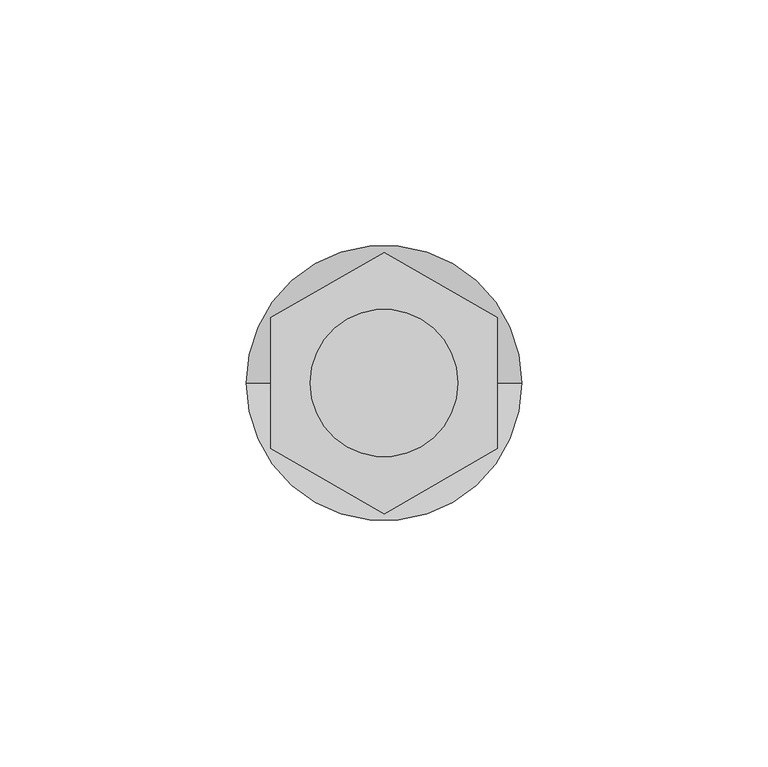
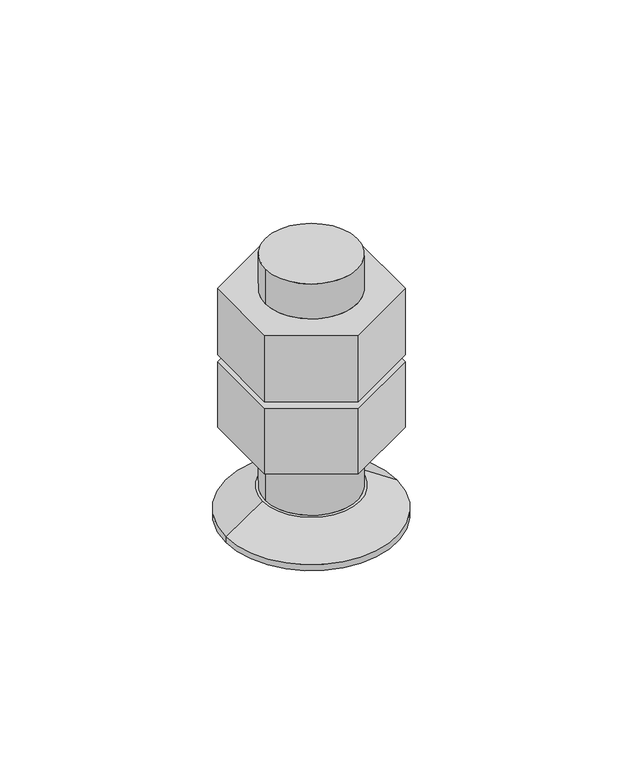
"""IFC4 building model written with IfcOpenShell, lengths in millimetres: fastener geometry, Bolt HPM-L : 30/L_mk."""

from ifc_helpers import new_model, si_unit, frame, origin, origin_with_axes, place, context, project, spatial, polyline, circle_curve, source, transform, mapped, element, save
from ifc_brep_helpers import plane_surface, cylinder_surface, revolved_surface, advanced_brep


def fastener_9f417b6c(model_context):
    return source(origin(), model_context, "Body", "AdvancedBrep", [
        advanced_brep(
        [(-23.0, -13.2790562, 22.7), (0.0, -26.5581124, 22.7), (23.0, -13.2790562, 22.7), (23.0, 13.2790562, 22.7), (0.0, 26.5581124, 22.7), (-23.0, 13.2790562, 22.7), (15.0, 0.0, 22.7), (-15.0, 0.0, 22.7), (-23.0, -13.2790562, 0.0), (-23.0, 13.2790562, 0.0), (0.0, 26.5581124, 0.0), (23.0, 13.2790562, 0.0), (23.0, -13.2790562, 0.0), (0.0, -26.5581124, 0.0), (-15.0, 0.0, 0.0), (15.0, 0.0, 0.0), (-15.0, 0.0, 60.0), (15.0, 0.0, 60.0), (15.0, 0.0, 48.0), (-15.0, 0.0, 48.0), (-15.0, 0.0, 25.0), (15.0, 0.0, 25.0), (15.0, 0.0, -20.0), (-15.0, 0.0, -20.0), (-23.0, -13.2790562, 48.0), (0.0, -26.5581124, 48.0), (23.0, -13.2790562, 48.0), (23.0, 13.2790562, 48.0), (0.0, 26.5581124, 48.0), (-23.0, 13.2790562, 48.0), (-23.0, -13.2790562, 25.0), (-23.0, 13.2790562, 25.0), (0.0, 26.5581124, 25.0), (23.0, 13.2790562, 25.0), (23.0, -13.2790562, 25.0), (0.0, -26.5581124, 25.0), (-28.0, 0.0, -30.0), (-28.0, 0.0, -28.0), (28.0, 0.0, -28.0), (28.0, 0.0, -30.0), (-16.0, 0.0, -20.0), (16.0, 0.0, -20.0)],
        [
            (0, 1),
            (1, 2),
            (2, 3),
            (3, 4),
            (4, 5),
            (5, 0),
            (6, 7, circle_curve(frame((0.0, 0.0, 22.7), z_axis=(0.0, 0.0, -1.0), x_axis=(1.0, 0.0, 0.0)), 15.0)),
            (7, 6, circle_curve(frame((0.0, 0.0, 22.7), z_axis=(0.0, 0.0, -1.0), x_axis=(1.0, 0.0, 0.0)), 15.0)),
            (8, 9),
            (9, 10),
            (10, 11),
            (11, 12),
            (12, 13),
            (13, 8),
            (14, 15, circle_curve(origin_with_axes(), 15.0)),
            (15, 14, circle_curve(origin_with_axes(), 15.0)),
            (5, 9),
            (8, 0),
            (4, 10),
            (3, 11),
            (2, 12),
            (1, 13),
            (16, 17, circle_curve(frame((0.0, 0.0, 60.0), z_axis=(0.0, 0.0, 1.0), x_axis=(1.0, 0.0, 0.0)), 15.0)),
            (17, 16, circle_curve(frame((0.0, 0.0, 60.0), z_axis=(0.0, 0.0, 1.0), x_axis=(1.0, 0.0, 0.0)), 15.0)),
            (17, 18),
            (18, 19, circle_curve(frame((0.0, 0.0, 48.0), z_axis=(0.0, 0.0, 1.0), x_axis=(1.0, 0.0, 0.0)), 15.0)),
            (19, 16),
            (7, 20),
            (20, 21, circle_curve(frame((0.0, 0.0, 25.0), z_axis=(0.0, 0.0, -1.0), x_axis=(1.0, 0.0, 0.0)), 15.0)),
            (21, 6),
            (15, 22),
            (22, 23, circle_curve(frame((0.0, 0.0, -20.0), z_axis=(0.0, 0.0, 1.0), x_axis=(1.0, 0.0, 0.0)), 15.0)),
            (23, 14),
            (19, 18, circle_curve(frame((0.0, 0.0, 48.0), z_axis=(0.0, 0.0, 1.0), x_axis=(1.0, 0.0, 0.0)), 15.0)),
            (21, 20, circle_curve(frame((0.0, 0.0, 25.0), z_axis=(0.0, 0.0, -1.0), x_axis=(1.0, 0.0, 0.0)), 15.0)),
            (23, 22, circle_curve(frame((0.0, 0.0, -20.0), z_axis=(0.0, 0.0, 1.0), x_axis=(1.0, 0.0, 0.0)), 15.0)),
            (24, 25),
            (25, 26),
            (26, 27),
            (27, 28),
            (28, 29),
            (29, 24),
            (30, 31),
            (31, 32),
            (32, 33),
            (33, 34),
            (34, 35),
            (35, 30),
            (29, 31),
            (30, 24),
            (28, 32),
            (27, 33),
            (26, 34),
            (25, 35),
            (36, 37),
            (37, 38, circle_curve(frame((0.0, 0.0, -28.0), z_axis=(0.0, 0.0, -1.0), x_axis=(1.0, 0.0, 0.0)), 28.0)),
            (38, 39),
            (39, 36, circle_curve(frame((0.0, 0.0, -30.0), z_axis=(0.0, 0.0, 1.0), x_axis=(1.0, 0.0, 0.0)), 28.0)),
            (38, 37, circle_curve(frame((0.0, 0.0, -28.0), z_axis=(0.0, 0.0, -1.0), x_axis=(1.0, 0.0, 0.0)), 28.0)),
            (36, 39, circle_curve(frame((0.0, 0.0, -30.0), z_axis=(0.0, 0.0, 1.0), x_axis=(1.0, 0.0, 0.0)), 28.0)),
            (40, 41, circle_curve(frame((0.0, 0.0, -20.0), z_axis=(0.0, 0.0, -1.0), x_axis=(1.0, 0.0, 0.0)), 16.0)),
            (41, 38),
            (37, 40),
            (41, 40, circle_curve(frame((0.0, 0.0, -20.0), z_axis=(0.0, 0.0, -1.0), x_axis=(-1.0, 0.0, 0.0)), 16.0)),
        ],
        [
            plane_surface(frame((-23.0, -13.2790562, 22.7), z_axis=(0.0, 0.0, 1.0), x_axis=(0.0, 1.0, 0.0))),
            plane_surface(frame((-23.0, -13.2790562, 0.0), z_axis=(0.0, 0.0, -1.0), x_axis=(0.0, -1.0, 0.0))),
            plane_surface(frame((-23.0, -13.2790562, 22.7), z_axis=(-1.0, 0.0, 0.0), x_axis=(0.0, 0.0, -1.0))),
            plane_surface(frame((-23.0, 13.2790562, 22.7), z_axis=(-0.4999999999999993, 0.8660254037844392, 0.0), x_axis=(0.0, 0.0, -1.0))),
            plane_surface(frame((0.0, 26.5581124, 22.7), z_axis=(0.5000000000000024, 0.8660254037844374, 0.0), x_axis=(0.0, 0.0, -1.0))),
            plane_surface(frame((23.0, 13.2790562, 22.7), z_axis=(1.0, 0.0, 0.0), x_axis=(0.0, 0.0, -1.0))),
            plane_surface(frame((23.0, -13.2790562, 22.7), z_axis=(0.4999999999999989, -0.8660254037844393, 0.0), x_axis=(0.0, 0.0, -1.0))),
            plane_surface(frame((0.0, -26.5581124, 22.7), z_axis=(-0.49999999999999895, -0.8660254037844393, 0.0), x_axis=(0.0, 0.0, -1.0))),
            plane_surface(frame((15.0, 0.0, 60.0), z_axis=(0.0, 0.0, 1.0), x_axis=(0.0, -1.0, 0.0))),
            cylinder_surface(frame((0.0, 0.0, -30.0), z_axis=(0.0, 0.0, 1.0), x_axis=(1.0, 0.0, 0.0)), 15.0),
            plane_surface(frame((-23.0, -13.2790562, 48.0), z_axis=(0.0, 0.0, 1.0), x_axis=(0.0, 1.0, 0.0))),
            plane_surface(frame((-23.0, -13.2790562, 25.0), z_axis=(0.0, 0.0, -1.0), x_axis=(0.0, -1.0, 0.0))),
            plane_surface(frame((-23.0, -13.2790562, 48.0), z_axis=(-1.0, 0.0, 0.0), x_axis=(0.0, 0.0, -1.0))),
            plane_surface(frame((-23.0, 13.2790562, 48.0), z_axis=(-0.4999999999999995, 0.866025403784439, 0.0), x_axis=(0.0, 0.0, -1.0))),
            plane_surface(frame((0.0, 26.5581124, 48.0), z_axis=(0.5000000000000024, 0.8660254037844373, 0.0), x_axis=(0.0, 0.0, -1.0))),
            plane_surface(frame((23.0, 13.2790562, 48.0), z_axis=(1.0, 0.0, 0.0), x_axis=(0.0, 0.0, -1.0))),
            plane_surface(frame((23.0, -13.2790562, 48.0), z_axis=(0.4999999999999991, -0.8660254037844393, 0.0), x_axis=(0.0, 0.0, -1.0))),
            plane_surface(frame((0.0, -26.5581124, 48.0), z_axis=(-0.49999999999999895, -0.8660254037844393, 0.0), x_axis=(0.0, 0.0, -1.0))),
            cylinder_surface(frame((0.0, 0.0, -30.0), z_axis=(0.0, 0.0, 1.0), x_axis=(1.0, 0.0, 0.0)), 28.0),
            revolved_surface(polyline([(16.000000021428573, 0.0, -20.0), (28.0, 0.0, -28.0)]), (0.0, 0.0, -9.3333333), (0.0, 0.0, -1.0)),
            revolved_surface(polyline([(-16.000000021428573, 0.0, -20.0), (-28.0, 0.0, -28.0)]), (0.0, 0.0, -9.3333333), (0.0, 0.0, -1.0)),
            plane_surface(frame((16.0, 0.0, -20.0), z_axis=(0.0, 0.0, 1.0), x_axis=(0.0, -1.0, 0.0))),
            plane_surface(frame((15.0, 0.0, -30.0), z_axis=(0.0, 0.0, -1.0), x_axis=(0.0, 1.0, 0.0))),
        ],
        [
            (0, [[1, 2, 3, 4, 5, 6], [7, 8]]),
            (1, [[9, 10, 11, 12, 13, 14], [15, 16]]),
            (2, [[17, -9, 18, -6]]),
            (3, [[19, -10, -17, -5]]),
            (4, [[20, -11, -19, -4]]),
            (5, [[21, -12, -20, -3]]),
            (6, [[22, -13, -21, -2]]),
            (7, [[-18, -14, -22, -1]]),
            (8, [[23, 24]]),
            (9, [[25, 26, 27, -24]]),
            (9, [[28, 29, 30, -8]]),
            (9, [[31, 32, 33, -16]]),
            (9, [[-27, 34, -25, -23]]),
            (9, [[-30, 35, -28, -7]]),
            (9, [[-33, 36, -31, -15]]),
            (10, [[37, 38, 39, 40, 41, 42], [-34, -26]]),
            (11, [[43, 44, 45, 46, 47, 48], [-35, -29]]),
            (12, [[49, -43, 50, -42]]),
            (13, [[51, -44, -49, -41]]),
            (14, [[52, -45, -51, -40]]),
            (15, [[53, -46, -52, -39]]),
            (16, [[54, -47, -53, -38]]),
            (17, [[-50, -48, -54, -37]]),
            (18, [[55, 56, 57, 58]]),
            (18, [[-57, 59, -55, 60]]),
            (19, [[61, 62, -56, 63]]),
            (20, [[-59, -62, 64, -63]]),
            (21, [[-64, -61], [-36, -32]]),
            (22, [[-58, -60]]),
        ],
    ),
    ])


if __name__ == "__main__":
    model = new_model("IFC4")
    model_context = context("Model", 3, world=origin())
    ifc_project = project(units=[si_unit("LENGTHUNIT", "METRE", prefix="MILLI")], contexts=[model_context])
    site = spatial("IfcSite", under=ifc_project)
    building = spatial("IfcBuilding", under=site)
    placement = place(None, origin())
    fastener_shape = fastener_9f417b6c(model_context)
    element("IfcFastener", 1, ObjectType="Bolt HPM-L : 30/L_mk", at=placement, inside=building, context=model_context, shape_type="MappedRepresentation", body=[
        mapped(fastener_shape, transform((0.0, 0.0, 0.0), x_axis=(1.0, 0.0, 0.0), y_axis=(0.0, 1.0, 0.0), z_axis=(0.0, 0.0, 1.0))),
    ])
    save(model, "model.ifc")

# Revit data of these elements
# Type "Bolt HPM-L : 30/L_mk"
#   Type Comments = "Mountingpart"
#   r3 = 15 mm
#   r2 = 28 mm
#   r1 = 16 mm
#   offset2 = 0 mm
#   l1 = 60 mm
#   Washer s = 8 mm
#   Washer Raduis2 = 32.5 mm
#   Washer Radius1 = 15.5 mm
#   Washer Diameter2 = 65 mm
#   Washer Diameter1 = 31 mm
#   T [instance default] = 45 mm
#   Offset1 [instance default] = 25 mm
#   Hexagonal nut m = 22.7 mm
#   l3 = 60 mm
#   l2 = 30 mm
#   hef = 20 mm
#   d3 = 30 mm
#   d1 = 32 mm
#   a = 90 mm
#   Hexagonal nut S1 = 23 mm
#   Hexagonal nut S = 46 mm
#   Material [instance default] = Metal - Steel - S355
#   Default Elevation = 0
# Element 1 (IfcFastener, "Bolt HPM-L : 30/L_mk")
#   Materials on its faces: "Metal - Steel - S355"
# Materials
#   "Metal - Steel - S355": class "Steel", colour RGB 247 247 247, transparency 0, Cost = 0
